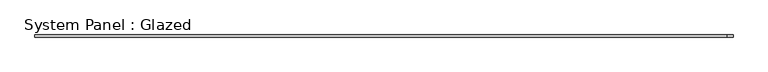
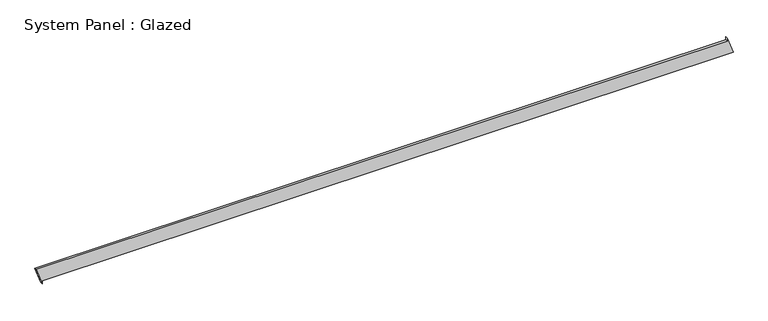
"""IFC4 building model written with IfcOpenShell, lengths in millimetres: plate geometry, System Panel : Glazed."""

from ifc_helpers import new_model, si_unit, frame, origin, place, context, project, spatial, polyline, outline, extrude, source, transform, mapped, element, save


def system_panel_glazed_c4fd97ea(model_context):
    return source(origin(), model_context, "Body", "SweptSolid", [
        extrude(outline(polyline([(0.0, -3958.7491356), (35.3553391, -3958.7491356), (35.3553391, 4028.0146093), (234.5559336, 3958.8677682), (199.2005945, 3958.8679874), (199.1510815, -4028.0146093), (0.0, -3958.7491356)])), frame((0.0, -49.5, 0.0), z_axis=(0.0, 1.0, 0.0), x_axis=(0.0, 0.0, 1.0)), (0.0, 0.0, 1.0), 25.0),
    ])


if __name__ == "__main__":
    model = new_model("IFC4")
    model_context = context("Model", 3, world=origin())
    ifc_project = project(units=[si_unit("LENGTHUNIT", "METRE", prefix="MILLI")], contexts=[model_context])
    site = spatial("IfcSite", under=ifc_project)
    building = spatial("IfcBuilding", under=site)
    placement = place(None, origin())
    system_panel_glazed_shape = system_panel_glazed_c4fd97ea(model_context)
    element("IfcPlate", 1, ObjectType="System Panel : Glazed", at=placement, inside=building, context=model_context, shape_type="MappedRepresentation", body=[
        mapped(system_panel_glazed_shape, transform((0.0, 0.0, 0.0), x_axis=(1.0, 0.0, 0.0), y_axis=(0.0, 1.0, 0.0), z_axis=(0.0, 0.0, 1.0))),
    ])
    save(model, "model.ifc")

# Revit data of these elements
# Element 1 (IfcPlate, "System Panel : Glazed")
#   Materials on its faces: "Glass"
# Materials
#   "Glass": class "Glass", colour RGB 218 227 224, transparency 0.85, Description = "Soda Lime Glass", Cost = 0
